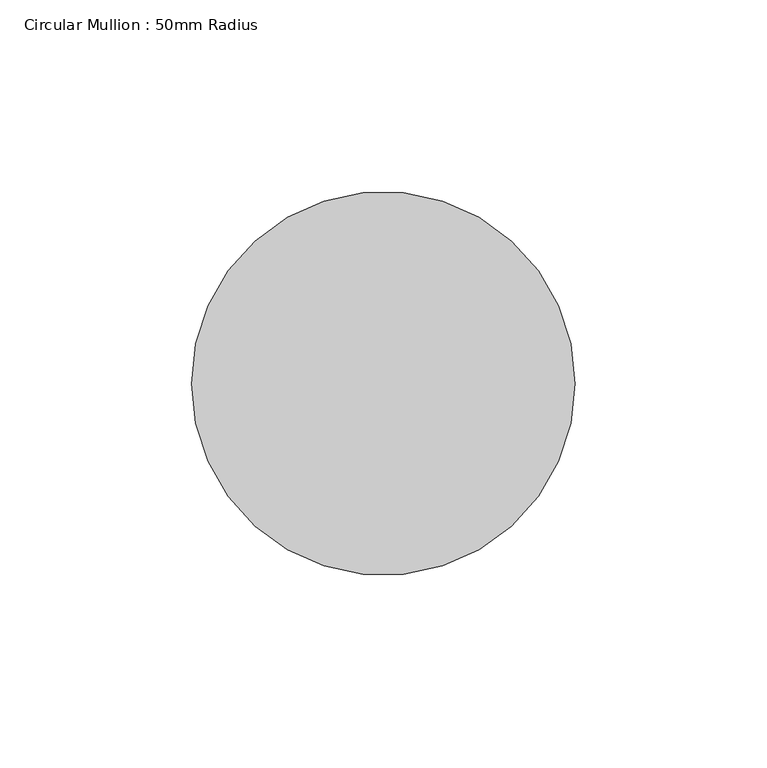
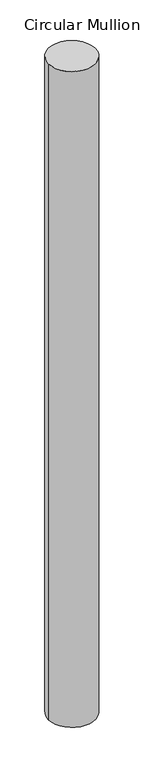
"""IFC4 building model written with IfcOpenShell, lengths in millimetres: member geometry, Circular Mullion : 50mm Radius."""

from ifc_helpers import new_model, si_unit, point, frame, origin, origin_2d, place, context, project, spatial, circle_curve, trimmed, segment, composite_curve, outline, extrude, source, transform, mapped, element, save


def circular_mullion_50mm_radius_25b05a63(model_context):
    return source(origin(), model_context, "Body", "SweptSolid", [
        extrude(outline(composite_curve([segment(trimmed(circle_curve(origin_2d(), 50.0), [point((50.0, 0.0))], [point((-50.0, 0.0))], False, "CARTESIAN"), True, "CONTINUOUS"), segment(trimmed(circle_curve(origin_2d(), 50.0), [point((-50.0, 0.0))], [point((50.0, 0.0))], False, "CARTESIAN"), True, "CONTINUOUS")], self_intersect=False)), frame((0.0, 0.0, -1480.2443483), z_axis=(0.0, 0.0, 1.0), x_axis=(1.0, 0.0, 0.0)), (0.0, 0.0, 1.0), 1480.2443483),
    ])


if __name__ == "__main__":
    model = new_model("IFC4")
    model_context = context("Model", 3, world=origin())
    ifc_project = project(units=[si_unit("LENGTHUNIT", "METRE", prefix="MILLI")], contexts=[model_context])
    site = spatial("IfcSite", under=ifc_project)
    building = spatial("IfcBuilding", under=site)
    placement = place(None, origin())
    circular_mullion_50mm_radius_shape = circular_mullion_50mm_radius_25b05a63(model_context)
    element("IfcMember", 1, ObjectType="Circular Mullion : 50mm Radius", at=placement, inside=building, context=model_context, shape_type="MappedRepresentation", body=[
        mapped(circular_mullion_50mm_radius_shape, transform((0.0, 0.0, 0.0), x_axis=(1.0, 0.0, 0.0), y_axis=(0.0, 1.0, 0.0), z_axis=(0.0, 0.0, 1.0))),
    ])
    save(model, "model.ifc")

# Revit data of these elements
# Type "Circular Mullion : 50mm Radius"
#   built-in parameter 1007350 = 0.164042 (stored number, unit not read)
# Element 1 (IfcMember, "Circular Mullion : 50mm Radius")
#   Materials on its faces: "Aluminium"
# Materials
#   "Aluminium": class "Metal", colour RGB 247 247 247, transparency 0, Description = "Aluminium 6061", Cost = 0
